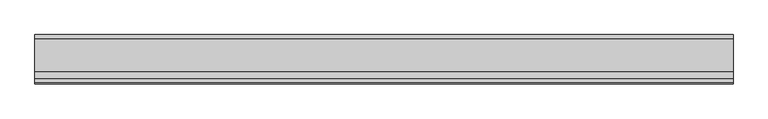
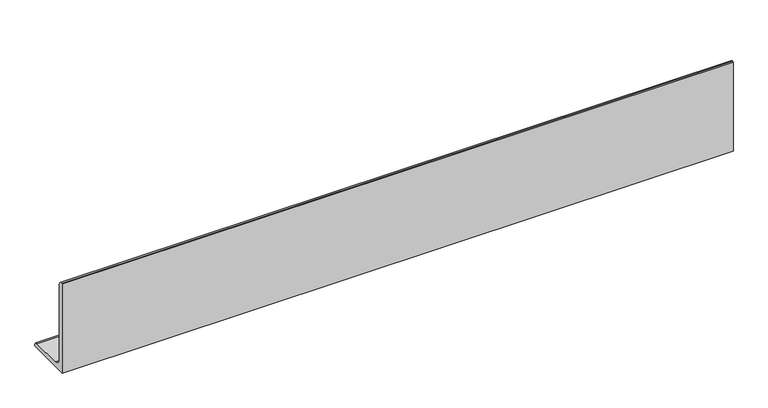
"""IFC4 building model written with IfcOpenShell, lengths in millimetres: beam geometry, NLRS_28_SF_LIB_stalen ligger hoekprofiel ongelijkzijdig-AV-MMBS-SRP_gen_rsf : stalen ligger ongelijzijdig hoekprofiel LUEQ_gen__200x100x10."""

from ifc_helpers import new_model, si_unit, point, frame, frame_2d, origin, place, context, project, spatial, polyline, circle_curve, trimmed, segment, composite_curve, outline, extrude, source, transform, mapped, element, save


def beam_4722c818(model_context):
    return source(origin(), model_context, "Body", "SweptSolid", [
        extrude(outline(composite_curve([segment(polyline([(-20.13, -69.3), (-20.13, 130.7), (-17.63, 130.7)]), True, "CONTINUOUS"), segment(trimmed(circle_curve(frame_2d((-17.63, 123.2)), 7.5), [point((-17.63, 130.7))], [point((-10.13, 123.2))], False, "CARTESIAN"), True, "CONTINUOUS"), segment(polyline([(-10.13, 123.2), (-10.13, -44.3)]), True, "CONTINUOUS"), segment(trimmed(circle_curve(frame_2d((4.87, -44.3)), 15.0), [point((-10.13, -44.3))], [point((4.87, -59.3))], True, "CARTESIAN"), True, "CONTINUOUS"), segment(polyline([(4.87, -59.3), (72.37, -59.3)]), True, "CONTINUOUS"), segment(trimmed(circle_curve(frame_2d((72.37, -66.8)), 7.5), [point((72.37, -59.3))], [point((79.87, -66.8))], False, "CARTESIAN"), True, "CONTINUOUS"), segment(polyline([(79.87, -66.8), (79.87, -69.3), (-20.13, -69.3)]), True, "CONTINUOUS")], self_intersect=False)), frame((-710.0, 0.0, 0.0), z_axis=(1.0, 0.0, 0.0), x_axis=(0.0, 1.0, 0.0)), (0.0, 0.0, 1.0), 1420.0),
    ])


if __name__ == "__main__":
    model = new_model("IFC4")
    model_context = context("Model", 3, world=origin())
    ifc_project = project(units=[si_unit("LENGTHUNIT", "METRE", prefix="MILLI")], contexts=[model_context])
    site = spatial("IfcSite", under=ifc_project)
    building = spatial("IfcBuilding", under=site)
    placement = place(None, origin())
    beam_shape = beam_4722c818(model_context)
    element("IfcBeam", 1, ObjectType="NLRS_28_SF_LIB_stalen ligger hoekprofiel ongelijkzijdig-AV-MMBS-SRP_gen_rsf : stalen ligger ongelijzijdig hoekprofiel LUEQ_gen__200x100x10", at=placement, inside=building, context=model_context, shape_type="MappedRepresentation", body=[
        mapped(beam_shape, transform((0.0, 0.0, 0.0), x_axis=(1.0, 0.0, 0.0), y_axis=(0.0, 1.0, 0.0), z_axis=(0.0, 0.0, 1.0))),
    ])
    save(model, "model.ifc")

# Revit data of these elements
# Type "NLRS_28_SF_LIB_stalen ligger hoekprofiel ongelijkzijdig-AV-MMBS-SRP_gen_rsf : stalen ligger ongelijzijdig hoekprofiel LUEQ_gen__200x100x10"
#   Type IfcGUID = "0dxhH9VHH5jh7XQ0uLfXuR"
#   IfcExportAs = "IfcBeamType"
#   Type Comments = "L200x100x10"
#   Model = " "
#   Manufacturer = " "
#   Fire Rating = " "
#   Description = "stalen ligger L200x100x10"
#   Assembly Code = "28.11"
#   vz = 130.7 mm
#   vy = 79.87 mm
#   tw = 10 mm
#   tf = 10 mm
#   ri = 7.5 mm
#   ra = 15 mm
#   d = 200 mm
#   bf = 100 mm
#   NLRS_C_lengte [instance default] = 1524 mm
#   Length [instance default] = 1524 mm
#   Structural Material = NLRS_h2_staal_gen_rsf
#   Keynote = ""
# Element 1 (IfcBeam, "NLRS_28_SF_LIB_stalen ligger hoekprofiel ongelijkzijdig-AV-MMBS-SRP_gen_rsf : stalen ligger ongelijzijdig hoekprofiel LUEQ_gen__200x100x10")
#   NLRS_C_lengte = 1420 mm
#   Materials on its faces: "NLRS_h2_staal_gen_rsf"
# Materials
#   "NLRS_h2_staal_gen_rsf": class "H - Metaal", colour RGB 189 187 185, transparency 0, Keynote = "h2", Manufacturer = "Revit Standards Foundation", URL = "www.revitstandards.org", Description = "staal", Cost = 0
